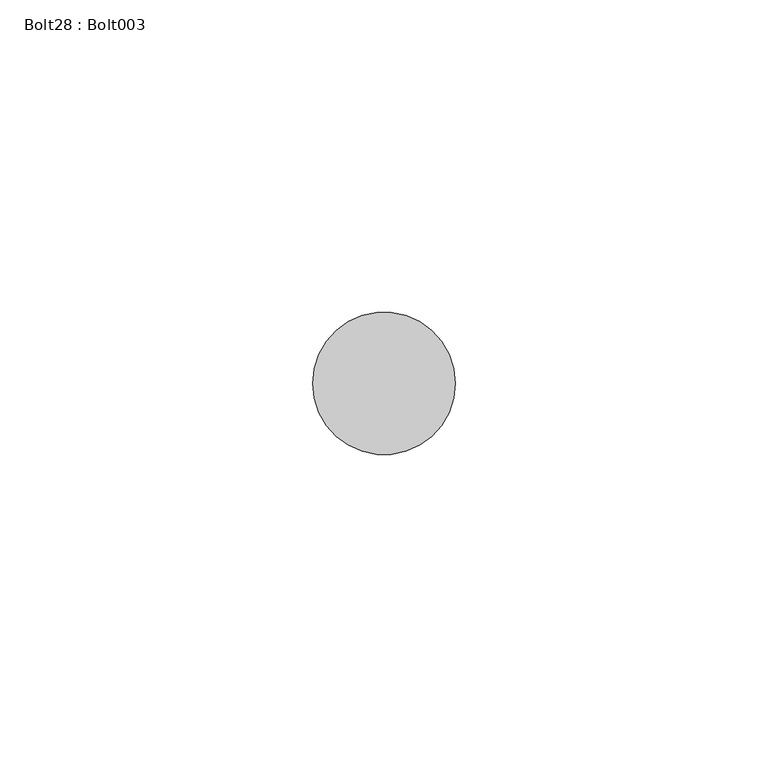
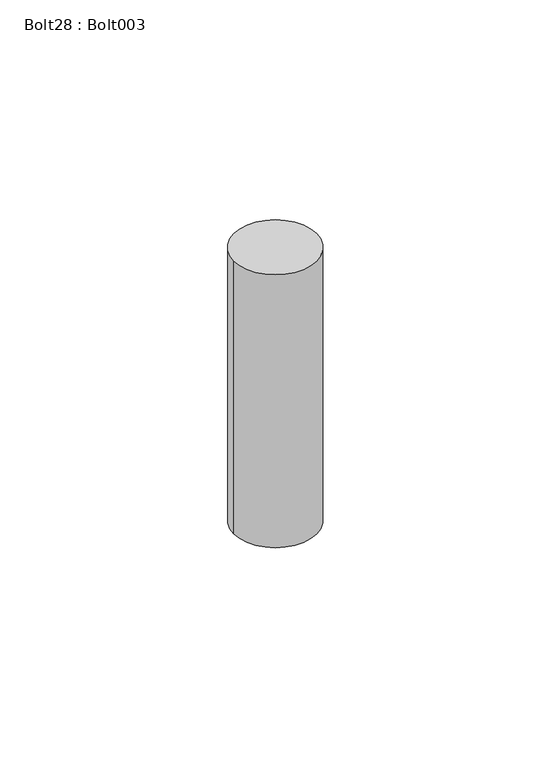
"""IFC4 building model written with IfcOpenShell, lengths in millimetres: proxy geometry, Bolt28 : Bolt003."""

from ifc_helpers import new_model, si_unit, point, frame, frame_2d, origin, place, context, project, spatial, circle_curve, trimmed, segment, composite_curve, outline, extrude, source, transform, mapped, element, save


def bolt28_bolt003_ef9ea109(model_context):
    return source(origin(), model_context, "Body", "SweptSolid", [
        extrude(outline(composite_curve([segment(trimmed(circle_curve(frame_2d((5062.3346014, 1896.5882072)), 11.4045168), [point((5073.7391183, 1896.5882072))], [point((5050.9300846, 1896.5882072))], False, "CARTESIAN"), True, "CONTINUOUS"), segment(trimmed(circle_curve(frame_2d((5062.3346014, 1896.5882072)), 11.4045168), [point((5050.9300846, 1896.5882072))], [point((5073.7391183, 1896.5882072))], False, "CARTESIAN"), True, "CONTINUOUS")], self_intersect=False)), frame((0.0, 0.0, 36645.5959962), z_axis=(0.0, 0.0, 1.0), x_axis=(1.0, 0.0, 0.0)), (0.0, 0.0, 1.0), 79.375),
    ])


if __name__ == "__main__":
    model = new_model("IFC4")
    model_context = context("Model", 3, world=origin())
    ifc_project = project(units=[si_unit("LENGTHUNIT", "METRE", prefix="MILLI")], contexts=[model_context])
    site = spatial("IfcSite", under=ifc_project)
    building = spatial("IfcBuilding", under=site)
    placement = place(None, origin())
    bolt28_bolt003_shape = bolt28_bolt003_ef9ea109(model_context)
    element("IfcBuildingElementProxy", 1, Name="Bolt28 : Bolt003", ObjectType="Bolt28 : Bolt003", at=placement, inside=building, context=model_context, shape_type="MappedRepresentation", body=[
        mapped(bolt28_bolt003_shape, transform((0.0, 0.0, 0.0), x_axis=(1.0, 0.0, 0.0), y_axis=(0.0, 1.0, 0.0), z_axis=(0.0, 0.0, 1.0))),
    ])
    save(model, "model.ifc")

# Revit data of these elements
# Type "Bolt28 : Bolt003"
#   NameOverride = "Bolt003"
# Element 1 (IfcBuildingElementProxy, "Bolt28 : Bolt003")
#   Materials on its faces: "STEEL ANGLE AND ANCHOR BOLT (SEE STRUCT. DWGS)"
# Materials
#   "STEEL ANGLE AND ANCHOR BOLT (SEE STRUCT. DWGS)": class "Unassigned", colour RGB 128 128 128, transparency 0, Cost = 0
